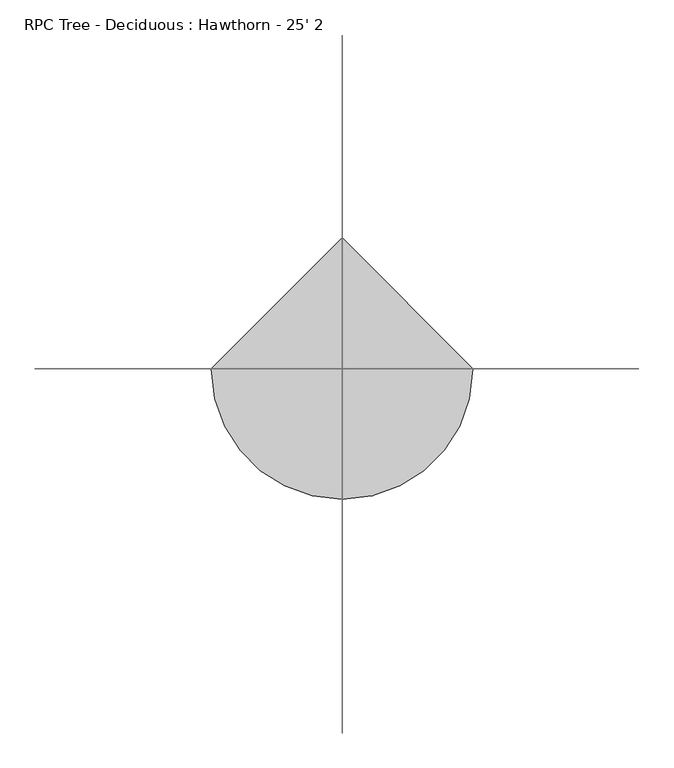
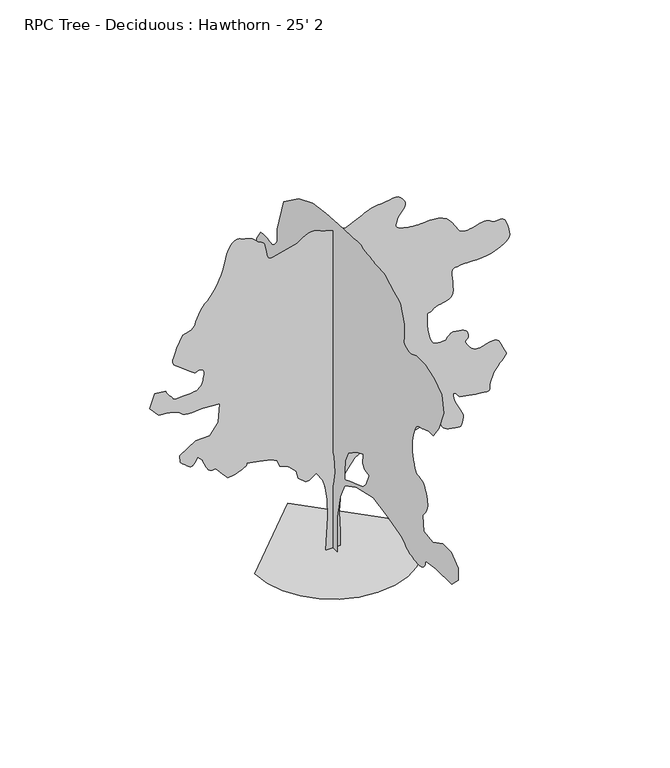
"""IFC4 building model written with IfcOpenShell, lengths in millimetres: geographic element geometry, RPC Tree - Deciduous : Hawthorn - 25' 2."""

from ifc_helpers import new_model, si_unit, origin, place, context, project, spatial, triangles, source, transform, mapped, element, save


def rpc_tree_deciduous_hawthorn_25_2_a438f522(model_context):
    return source(origin(), model_context, "Body", "Tessellation", [
        triangles([(159.1331283, 0.0003947, 0.019308), (-154.090976, 0.0003947, 0.019308), (-109.3440979, 0.0003507, 738.3315319), (-120.5310059, 0.000328, 1118.6758307), (-165.2768666, 0.0003107, 1409.5258827), (-210.0237538, 0.0003, 1588.5119053), (-355.4472356, 0.000288, 1789.8701088), (-500.8748051, 0.000294, 1689.1897717), (-579.1803815, 0.0002947, 1678.0035358), (-735.7915707, 0.0002867, 1812.2424351), (-780.538694, 0.000276, 1991.2284576), (-937.1498468, 0.0002667, 2147.8396832), (-1127.3219599, 0.000262, 2226.1452232), (-1183.2552464, 0.000254, 2360.3841225), (-1306.3080551, 0.00025, 2427.5035721), (-1563.5970016, 0.0002467, 2483.4367859), (-1820.8885643, 0.000244, 2528.1814384), (-1818.86674, 0.0002446, 2518.4962738), (-1819.0953598, 0.0002452, 2508.2221916), (-1823.8248676, 0.0002459, 2496.7743439), (-1835.3057076, 0.0002466, 2483.5664291), (-1855.7857075, 0.0002476, 2468.0089485), (-1887.5203983, 0.0002487, 2449.5176353), (-1932.7551373, 0.00025, 2427.5035721), (-1983.2071449, 0.0002513, 2406.1420853), (-2029.5519905, 0.0002523, 2389.4746433), (-2072.4703011, 0.000253, 2376.7238228), (-2112.6530228, 0.0002536, 2367.102317), (-2150.7784573, 0.000254, 2359.8303772), (-2187.5321732, 0.0002544, 2354.1230221), (-2223.605262, 0.0002547, 2349.1978867), (-2346.6579254, 0.0002467, 2483.4367859), (-2480.8968246, 0.0002373, 2640.0478661), (-2507.2492859, 0.0002376, 2635.5522102), (-2533.5026253, 0.0002377, 2632.8090637), (-2559.5553955, 0.0002377, 2633.596225), (-2585.33638, 0.0002373, 2639.6670753), (-2610.710994, 0.0002366, 2652.7732521), (-2635.5774994, 0.0002353, 2674.6934258), (-2659.885318, 0.0002333, 2707.1548164), (-2681.9072296, 0.0002311, 2744.2133102), (-2700.3982521, 0.000229, 2778.9097389), (-2715.9429428, 0.0002271, 2811.6501823), (-2729.1511482, 0.0002252, 2842.8413017), (-2740.6065536, 0.0002234, 2872.8385986), (-2750.8681366, 0.0002217, 2902.0740234), (-2760.570742, 0.00022, 2930.9030777), (-2861.2308769, 0.000214, 3031.5885017), (-2928.3631165, 0.00022, 2930.9030777), (-2940.4789467, 0.0002211, 2912.005394), (-2953.5089653, 0.0002221, 2894.8857994), (-2968.2664948, 0.0002229, 2881.2968033), (-2985.6907219, 0.0002234, 2872.9656258), (-3006.6202583, 0.0002235, 2871.6956451), (-3031.9695831, 0.0002231, 2879.2396614), (-3062.6020157, 0.000222, 2897.3496025), (-3096.5362816, 0.0002205, 2923.0035599), (-3130.1150459, 0.0002188, 2950.6387917), (-3161.5093506, 0.0002172, 2978.0708382), (-3189.0175552, 0.0002157, 3003.1405289), (-3210.8362816, 0.0002144, 3023.7145638), (-3225.212439, 0.0002136, 3037.6337723), (-3230.3940994, 0.0002133, 3042.7645638), (-3241.5701614, 0.000204, 3199.3808762), (-2905.9857033, 0.0001913, 3411.9277863), (-2603.9547203, 0.0001906, 3423.1038483), (-2424.9634655, 0.0001766, 3658.0281715), (-2391.402578, 0.0001526, 4060.7448692), (-2760.570742, 0.0001506, 4094.2980537), (-2839.3868614, 0.0001512, 4085.027108), (-2916.5522095, 0.0001516, 4077.7374367), (-2990.3898537, 0.0001518, 4074.3338654), (-3059.2490227, 0.0001517, 4076.8229576), (-3121.4283669, 0.0001511, 4087.1354095), (-3175.301532, 0.0001499, 4107.2266251), (-3219.2180374, 0.000148, 4139.0528801), (-3263.4394661, 0.0001459, 4173.1650421), (-3318.227401, 0.0001444, 4199.6317406), (-3381.8287514, 0.0001432, 4219.7741158), (-3452.4660095, 0.0001423, 4234.8106979), (-3528.3866661, 0.0001416, 4246.0120491), (-3607.8379211, 0.0001411, 4254.6990189), (-3689.0413948, 0.0001406, 4262.0904282), (-3879.2111824, 0.000128, 4474.6373383), (-3767.3496964, 0.0001106, 4765.4925499), (-3543.6267242, 0.000112, 4743.1151367), (-3529.174118, 0.0001135, 4716.8007545), (-3514.3404305, 0.0001151, 4690.7657158), (-3498.7195816, 0.0001166, 4665.3402328), (-3481.9046196, 0.0001181, 4640.7786507), (-3463.5406242, 0.0001195, 4617.3853111), (-3443.2206436, 0.0001208, 4595.4904266), (-3420.563887, 0.000122, 4575.3227623), (-3403.5713196, 0.0001231, 4556.2983421), (-3395.5956436, 0.0001242, 4538.2642685), (-3389.1692917, 0.0001251, 4522.1861801), (-3376.875856, 0.0001259, 4509.0544235), (-3351.2727676, 0.0001265, 4499.8340561), (-3304.9177483, 0.0001267, 4495.4907166), (-3230.3940994, 0.0001266, 4497.0147514), (-3147.7933273, 0.0001263, 4501.8153305), (-3080.4326134, 0.0001261, 4506.6159096), (-3025.7972855, 0.0001258, 4511.3911995), (-2981.3473824, 0.0001255, 4516.1917786), (-2944.5429428, 0.0001252, 4520.9923576), (-2912.7928459, 0.0001249, 4525.7929367), (-2883.6082901, 0.0001246, 4530.5679359), (-2855.0332901, 0.0001233, 4552.2596352), (-2827.6521126, 0.000122, 4574.6370483), (-2802.607711, 0.0001206, 4598.3858894), (-2781.0686188, 0.0001191, 4624.1668739), (-2764.2539474, 0.0001174, 4652.7165848), (-2753.2810707, 0.0001154, 4684.6695763), (-2749.3693909, 0.0001133, 4720.7377235), (-2745.4071327, 0.0001109, 4760.7934181), (-2736.720163, 0.0001084, 4802.805098), (-2728.2366692, 0.0001059, 4844.6133018), (-2724.858387, 0.0001036, 4884.0850204), (-2731.4370552, 0.0001015, 4919.0352127), (-2752.8999893, 9.98e-05, 4947.3561584), (-2794.1242172, 9.86e-05, 4966.8636887), (-2835.4754723, 9.84e-05, 4971.2320267), (-2860.596032, 9.89e-05, 4962.0883987), (-2879.2396614, 9.97e-05, 4949.2356949), (-2901.2359932, 0.0001001, 4942.4541321), (-2936.3132126, 9.95e-05, 4951.5216019), (-2994.3015335, 9.75e-05, 4986.2183212), (-3084.9794289, 9.33e-05, 5056.3477615), (-3185.5886948, 8.86e-05, 5134.4522964), (-3266.6398521, 8.52e-05, 5192.2121429), (-3327.7268211, 8.25e-05, 5238.0337646), (-3368.4429405, 7.99e-05, 5280.3497864), (-3388.4327087, 7.71e-05, 5327.5178375), (-3387.2897552, 7.35e-05, 5388.0205399), (-3364.6329987, 6.86e-05, 5470.2399399), (-3332.3750839, 6.34e-05, 5558.3020065), (-3302.4792343, 5.9e-05, 5632.2666779), (-3274.5137901, 5.53e-05, 5694.4966003), (-3248.1488297, 5.21e-05, 5747.3282593), (-3222.926532, 4.94e-05, 5793.1248825), (-3198.4916862, 4.69e-05, 5834.2217926), (-3174.4635017, 4.46e-05, 5872.9566376), (-3129.0991196, 4.4e-05, 5882.81185), (-3084.8015327, 4.34e-05, 5894.2163864), (-3042.6628258, 4.25e-05, 5908.7707306), (-3003.7500847, 4.13e-05, 5928.0236252), (-2969.155394, 3.98e-05, 5953.5255569), (-2939.945549, 3.78e-05, 5986.850267), (-2917.1617653, 3.53e-05, 6029.5732407), (-2900.9310699, 3.27e-05, 6072.7020035), (-2888.6120544, 3.06e-05, 6108.7701508), (-2877.258387, 2.86e-05, 6141.7140701), (-2863.9487343, 2.66e-05, 6175.4195709), (-2845.7370552, 2.43e-05, 6213.8497833), (-2819.7273056, 2.15e-05, 6260.8649368), (-2782.9228661, 1.79e-05, 6320.4281616), (-2744.5688118, 1.47e-05, 6374.7841461), (-2713.0727692, 1.26e-05, 6410.1918686), (-2684.3201637, 1.1e-05, 6436.3792236), (-2654.1702599, 9.4e-06, 6463.150264), (-2618.5596428, 7.2e-06, 6500.2852066), (-2573.3475769, 3.8e-06, 6557.5875229), (-2514.4552414, -1.4e-06, 6644.8362671), (-2453.8586494, -7.4e-06, 6746.4620407), (-2405.0042187, -1.31e-05, 6841.4324066), (-2365.9314583, -1.85e-05, 6931.32285), (-2334.6868538, -2.36e-05, 7017.682695), (-2309.3123852, -2.86e-05, 7102.0868454), (-2287.8543926, -3.36e-05, 7186.1102051), (-2268.3497692, -3.87e-05, 7271.2759369), (-2244.5754936, -4.38e-05, 7356.7980423), (-2212.386034, -4.86e-05, 7437.6204346), (-2172.9551559, -5.29e-05, 7509.0451447), (-2127.4586597, -5.63e-05, 7566.3730408), (-2077.0701656, -5.86e-05, 7604.9299896), (-2022.9657646, -5.95e-05, 7619.9924423), (-1966.3136993, -5.87e-05, 7606.8862656), (-1910.121199, -5.73e-05, 7582.9086594), (-1856.4689507, -5.63e-05, 7565.7887741), (-1805.1685936, -5.54e-05, 7551.412326), (-1756.0195587, -5.45e-05, 7535.6644501), (-1708.8265091, -5.32e-05, 7514.4302811), (-1663.3961426, -5.14e-05, 7483.5943726), (-1619.5303608, -4.87e-05, 7439.0936005), (-1579.0555058, -4.63e-05, 7399.0890656), (-1543.670747, -4.51e-05, 7378.0827896), (-1512.9800331, -4.44e-05, 7366.2974625), (-1486.5970505, -4.37e-05, 7353.9022888), (-1464.1256023, -4.23e-05, 7331.1437943), (-1445.1773403, -3.97e-05, 7288.217926), (-1429.3581024, -3.54e-05, 7215.3456299), (-1415.9875523, -3.04e-05, 7132.3890656), (-1403.2038849, -2.64e-05, 7065.2571167), (-1388.8528713, -2.34e-05, 7013.4155136), (-1370.7858055, -2.11e-05, 6976.2299927), (-1346.8464237, -1.98e-05, 6953.1412857), (-1314.8855839, -1.92e-05, 6943.5401276), (-1272.7470222, -1.94e-05, 6946.8678314), (-758.1663677, -2.74e-05, 7081.1067307), (-698.2198814, -2.99e-05, 7123.7785446), (-638.1794329, -3.23e-05, 7163.5040268), (-577.9408496, -3.43e-05, 7197.3368454), (-517.4101693, -3.58e-05, 7222.4068268), (-456.4857994, -3.66e-05, 7235.6908997), (-395.0737412, -3.65e-05, 7234.3444702), (-333.0749456, -3.54e-05, 7215.3456299), (-271.7289263, -3.38e-05, 7188.8786407), (-212.1431193, -3.25e-05, 7166.5015182), (-154.0251915, -3.14e-05, 7147.5526749), (-97.0814925, -3.04e-05, 7131.34785), (-41.0181631, -2.95e-05, 7117.1742966), (14.4578691, -2.88e-05, 7104.3983322), (69.6403804, -2.81e-05, 7092.3077911), (270.9999556, -2.67e-05, 7069.9306686), (584.2222612, -3.47e-05, 7204.1695679), (629.9473045, -3.64e-05, 7232.7445679), (676.749317, -3.81e-05, 7260.1254547), (725.7026516, -3.96e-05, 7285.1698563), (777.8843502, -4.08e-05, 7306.7092392), (834.371382, -4.18e-05, 7323.5239105), (896.2406433, -4.25e-05, 7334.4964966), (964.56656, -4.27e-05, 7338.4084671), (1038.7294024, -4.3e-05, 7343.6912842), (1115.4373655, -4.38e-05, 7356.0102997), (1191.7540735, -4.46e-05, 7370.107695), (1264.743441, -4.52e-05, 7380.6739105), (1331.4717808, -4.54e-05, 7382.4261292), (1389.0027168, -4.46e-05, 7370.107695), (1434.402562, -4.27e-05, 7338.4084671), (1469.8203129, -4.03e-05, 7297.1080811), (1498.5858536, -3.8e-05, 7258.7540268), (1519.5229477, -3.58e-05, 7222.177771), (1531.4610271, -3.37e-05, 7186.1607834), (1533.2212395, -3.15e-05, 7149.5595291), (1523.6327259, -2.92e-05, 7111.2054749), (1501.5195408, -2.67e-05, 7069.9306686), (1474.1255733, -2.45e-05, 7032.3637756), (1449.4698109, -2.28e-05, 7003.585881), (1427.5522533, -2.14e-05, 6980.1163834), (1408.3752262, -2.01e-05, 6958.3991043), (1391.9388748, -1.87e-05, 6934.9040268), (1378.2407284, -1.7e-05, 6906.151712), (1367.2806416, -1.47e-05, 6868.5598206), (1355.7362881, -1.23e-05, 6828.0210159), (1343.4097149, -1.02e-05, 6792.1819244), (1334.9946762, -8.3e-06, 6760.2542221), (1335.1903038, -6.6e-06, 6731.4507477), (1348.692968, -5e-06, 6705.0093384), (1380.1965683, -3.5e-06, 6680.1172531), (1434.402562, -2.1e-06, 6656.0123291), (1502.5633724, -8e-07, 6635.3118484), (1571.509164, 1e-07, 6620.4778702), (1639.2813354, 7e-07, 6610.5209198), (1703.9217213, 1e-06, 6604.5015198), (1763.4744816, 1.2e-06, 6601.4028717), (1815.9839218, 1.3e-06, 6600.2593369), (1859.4914406, 1.3e-06, 6600.0820221), (1908.6404755, 1.1e-06, 6602.7998795), (1975.9885448, 8e-07, 6608.0571167), (2056.4454071, 6e-07, 6611.5371368), (2144.9261982, 8e-07, 6608.9715958), (2236.3432926, 1.5e-06, 6596.0177353), (2325.6064487, 3.2e-06, 6568.3827942), (2407.633128, 5.9e-06, 6521.7734299), (2476.0555504, 9.6e-06, 6460.1789337), (2530.3911873, 1.36e-05, 6393.2754593), (2574.3635033, 1.77e-05, 6325.4063461), (2611.6760513, 2.15e-05, 6260.8649368), (2646.0422676, 2.49e-05, 6203.9689911), (2681.1959358, 2.76e-05, 6158.9856903), (2720.8452599, 2.93e-05, 6130.258374), (2765.3207428, 3.01e-05, 6115.9580841), (2812.1074219, 3.05e-05, 6110.4973709), (2860.8753754, 3.04e-05, 6112.3513275), (2911.1926529, 2.99e-05, 6120.0729492), (2962.6784637, 2.92e-05, 6132.2140686), (3014.9770157, 2.83e-05, 6147.2765213), (3067.6310692, 2.73e-05, 6163.8115585), (3115.4592545, 2.67e-05, 6173.1080841), (3162.4746986, 2.63e-05, 6180.6518097), (3207.9405281, 2.6e-05, 6184.6649368), (3251.0698723, 2.61e-05, 6183.3952469), (3291.0494087, 2.66e-05, 6175.0637787), (3327.1172653, 2.76e-05, 6157.9444748), (3358.4862808, 2.93e-05, 6130.258374), (3393.4620529, 3.05e-05, 6109.9386841), (3438.1912994, 3.06e-05, 6108.7957306), (3488.8135002, 3.01e-05, 6115.881926), (3541.3913956, 2.99e-05, 6120.200267), (3592.0135963, 3.04e-05, 6110.8531631), (3636.7428429, 3.25e-05, 6076.8424484), (3671.718615, 3.66e-05, 6007.1955368), (3699.2776886, 4.18e-05, 5920.2258453), (3722.3408157, 4.65e-05, 5841.4608856), (3737.75877, 5.07e-05, 5770.9250748), (3742.4323219, 5.44e-05, 5708.5934143), (3733.1866653, 5.76e-05, 5654.4914841), (3706.9484413, 6.04e-05, 5608.5937042), (3660.5172638, 6.26e-05, 5570.9256546), (3605.0439056, 6.46e-05, 5537.5247864), (3550.9419754, 6.65e-05, 5505.1145554), (3494.096608, 6.84e-05, 5474.6594376), (3430.3935196, 7e-05, 5447.1262344), (3355.7431343, 7.14e-05, 5423.5044205), (3266.0302963, 7.25e-05, 5404.7846329), (3157.1407219, 7.33e-05, 5391.931929), (3050.6893707, 7.37e-05, 5385.4549988), (2967.1235413, 7.38e-05, 5383.8550964), (2900.6008575, 7.37e-05, 5385.2009445), (2845.2036575, 7.36e-05, 5387.5124313), (2795.1148544, 7.35e-05, 5388.8332809), (2744.4417847, 7.36e-05, 5387.2327972), (2687.2917847, 7.4e-05, 5380.755867), (2632.1995079, 7.44e-05, 5373.8725662), (2590.4418823, 7.46e-05, 5369.5292267), (2560.1905312, 7.5e-05, 5363.4330872), (2539.7510811, 7.57e-05, 5351.2663879), (2527.325386, 7.71e-05, 5328.7369492), (2521.1609367, 7.93e-05, 5291.5258484), (2519.4970848, 8.26e-05, 5235.3409058), (2523.9979729, 8.71e-05, 5159.8269104), (2533.5866318, 9.23e-05, 5072.4002701), (2542.3849319, 9.78e-05, 4980.2494995), (2544.5441025, 0.0001032, 4890.6636887), (2534.1732239, 0.0001079, 4810.8569321), (2505.4078285, 0.0001117, 4748.0680321), (2452.3776352, 0.000114, 4709.5616615), (2387.9658691, 0.0001152, 4689.2416809), (2328.8373562, 0.0001161, 4674.4079933), (2274.7963234, 0.0001168, 4662.2924538), (2225.6474339, 0.0001175, 4650.2019127), (2181.1949146, 0.0001184, 4635.3682251), (2141.2406673, 0.0001196, 4615.0482445), (2105.594442, 0.0001213, 4586.4988243), (2074.7410927, 0.0001226, 4564.2231491), (2049.1734673, 0.000123, 4557.6189011), (2028.6908512, 0.0001231, 4556.2727623), (2013.1029945, 0.0001235, 4549.846701), (2002.2088921, 0.0001248, 4527.9773964), (1995.8156776, 0.0001276, 4480.2506584), (1993.727869, 0.0001326, 4396.3293274), (1998.2947414, 0.000139, 4289.0143661), (2011.0810249, 0.0001454, 4181.4709305), (2030.7126755, 0.0001515, 4079.0327065), (2055.8256775, 0.000157, 3986.9578033), (2085.0483124, 0.0001616, 3910.5546181), (2117.0091522, 0.0001649, 3855.0812599), (2150.3415653, 0.0001666, 3825.8202553), (2188.6294899, 0.0001673, 3814.6444839), (2233.3766132, 0.0001676, 3808.9294258), (2280.0795765, 0.0001677, 3807.3292328), (2324.2399624, 0.0001677, 3808.4721863), (2361.351796, 0.0001675, 3810.9868584), (2386.9220375, 0.0001674, 3813.5015305), (2396.4468922, 0.0001673, 3814.6444839), (2400.0004543, 0.0001668, 3823.2041359), (2411.1865448, 0.0001655, 3844.8958351), (2430.787674, 0.0001638, 3873.6231514), (2459.5862068, 0.000162, 3903.3411049), (2498.3643631, 0.0001605, 3927.9791359), (2547.8968048, 0.0001597, 3941.4411049), (2608.9837738, 0.00016, 3937.6817413), (2671.9758591, 0.0001607, 3924.8296188), (2726.5347382, 0.0001614, 3912.9675522), (2772.483387, 0.0001623, 3898.9468964), (2809.6183296, 0.0001634, 3879.6428421), (2837.7866684, 0.0001651, 3851.906163), (2856.7352211, 0.0001674, 3812.6379204), (2866.2855103, 0.0001706, 3758.7135956), (2862.7040428, 0.0001735, 3709.9456421), (2847.1593521, 0.0001752, 3682.3104103), (2826.9411095, 0.0001761, 3666.8418777), (2809.2625374, 0.0001769, 3654.4722839), (2801.3885994, 0.0001779, 3636.235025), (2810.5072289, 0.0001799, 3603.1387894), (2843.9080971, 0.0001833, 3546.1666855), (2889.3486374, 0.000187, 3484.6480568), (2930.6490234, 0.0001895, 3441.7218979), (2969.2315521, 0.0001912, 3414.061377), (3006.467942, 0.0001921, 3398.3640793), (3043.6790428, 0.0001925, 3391.2523041), (3082.2615715, 0.0001926, 3389.4233459), (3123.5619576, 0.0001926, 3389.5503731), (3174.7428452, 0.0001921, 3399.3294273), (3238.4459335, 0.0001908, 3421.249601), (3309.3628258, 0.0001894, 3444.134832), (3382.2607018, 0.0001886, 3456.860218), (3451.8311646, 0.0001891, 3448.2496971), (3512.7911064, 0.0001916, 3407.1524963), (3559.8571289, 0.0001966, 3322.4181335), (3596.9920715, 0.0002022, 3228.6924591), (3629.6310677, 0.0002061, 3162.9572273), (3654.6498894, 0.0002089, 3117.5419762), (3668.8993103, 0.0002108, 3084.8776909), (3669.2803917, 0.0002124, 3057.2680389), (3652.5924568, 0.0002142, 3027.1437149), (3615.7880173, 0.0002166, 2986.8336754), (3572.5063568, 0.0002193, 2942.3837723), (3537.6831917, 0.0002217, 2904.233194), (3509.8447746, 0.0002237, 2871.3148544), (3487.6196777, 0.0002256, 2842.5872475), (3469.6111839, 0.0002272, 2817.0094482), (3454.4219948, 0.0002288, 2793.5399506), (3440.6298134, 0.0002303, 2771.0863792), (3437.2006622, 0.00023, 2773.5501823), (3432.5271103, 0.0002299, 2772.1278854), (3425.3897552, 0.0002303, 2763.0345451), (3414.5439056, 0.0002314, 2742.4099319), (3398.7451607, 0.0002335, 2706.4182335), (3376.7235397, 0.0002367, 2651.1986389), (3347.3102188, 0.0002413, 2572.9412064), (3325.1359909, 0.0002461, 2493.0582916), (3319.1924583, 0.0002496, 2433.9271626), (3319.7005669, 0.000252, 2392.9976841), (3316.9065514, 0.0002535, 2367.722192), (3300.9807793, 0.0002543, 2355.5581089), (3262.1694855, 0.0002544, 2353.9579159), (3190.6939064, 0.000254, 2360.3841225), (3103.5213203, 0.0002534, 2370.2977615), (3023.3843513, 0.0002528, 2380.8006088), (2949.1147568, 0.0002521, 2391.791217), (2879.544294, 0.0002514, 2403.1729351), (2813.5044296, 0.0002507, 2414.8492573), (2749.8266304, 0.00025, 2426.721207), (2687.2917847, 0.0002493, 2438.6895172), (2647.0584846, 0.0002464, 2487.937674), (2609.8473839, 0.0002438, 2530.6275101), (2578.6815536, 0.0002421, 2560.2158203), (2556.6343529, 0.0002415, 2570.1219017), (2546.7285622, 0.0002425, 2553.8150482), (2551.9863808, 0.0002454, 2504.7319977), (2575.4302986, 0.0002507, 2416.3173363), (2612.9463226, 0.0002568, 2313.8436493), (2654.9324226, 0.000262, 2225.2638817), (2696.3598358, 0.0002666, 2148.0351654), (2732.09748, 0.0002707, 2079.6102722), (2757.0910126, 0.0002744, 2017.4488049), (2766.209642, 0.0002779, 1959.0060059), (2754.4240242, 0.0002813, 1901.734211), (2736.8980591, 0.0002844, 1850.8910934), (2728.0081947, 0.0002866, 1812.7631882), (2721.2516304, 0.0002882, 1786.3802055), (2710.2025955, 0.0002891, 1770.7567406), (2688.3841599, 0.0002895, 1764.9197422), (2649.3443916, 0.0002893, 1767.8864216), (2586.6063606, 0.0002887, 1778.6815475), (2516.4972679, 0.0002878, 1792.6413059), (2458.5092377, 0.000287, 1806.7966919), (2411.0875683, 0.000286, 1822.7122902), (2372.6700005, 0.0002849, 1841.9528309), (2341.6871532, 0.0002834, 1866.0878403), (2316.5741512, 0.0002816, 1896.6795776), (2295.766555, 0.0002793, 1935.2952438), (2282.6220085, 0.0002768, 1976.9435738), (2278.2862267, 0.0002746, 2015.0688629), (2277.8621246, 0.0002726, 2048.8888916), (2276.46003, 0.0002708, 2077.6214401), (2269.185474, 0.0002695, 2100.4838528), (2251.1515457, 0.0002685, 2116.6915844), (2217.4610149, 0.000268, 2125.4673569), (2177.5728973, 0.0002678, 2129.2823856), (2143.5572411, 0.0002676, 2131.3372021), (2114.4335827, 0.0002676, 2131.9239395), (2089.2216042, 0.0002676, 2131.3372021), (2066.9483997, 0.0002677, 2129.8691231), (2046.6284191, 0.0002678, 2127.8143066), (2027.2887566, 0.000268, 2125.4673569), (1758.8111034, 0.000274, 2024.7868744), (1579.8250809, 0.0002667, 2147.8396832), (1380.9128036, 0.0002704, 2075.457328), (1410.85429, 0.0002716, 2057.3014595), (1436.60984, 0.0002729, 2038.5130714), (1453.9936626, 0.0002741, 2018.4597897), (1458.8195309, 0.0002755, 1996.5066238), (1446.9019444, 0.0002771, 1972.0210545), (1414.0572922, 0.0002788, 1944.370562), (1356.0970219, 0.0002807, 1912.9203014), (1293.4784603, 0.0002823, 1885.3308517), (1245.5334217, 0.0002833, 1868.8920296), (1206.3972204, 0.0002837, 1862.4353016), (1170.1971771, 0.0002835, 1864.7822514), (1131.0609032, 0.0002829, 1874.7644909), (1083.118408, 0.0002819, 1891.2008423), (1020.4998465, 0.0002807, 1912.9203014), (729.6473236, 0.0002753, 2002.4145481), (461.1695615, 0.000284, 1856.9895584), (259.8112671, 0.0003, 1588.5119053), (192.6930892, 0.0003113, 1398.3397923), (170.3192732, 0.0003253, 1163.422954), (136.7603205, 0.0003487, 771.8924921), (159.1331283, 0.0003767, 302.0564901), (-0.000123, -157.488225, 0.0160584), (-0.000123, 166.924822, 0.0160778), (-0.0001013, 177.738606, 702.9113102), (-8.68e-05, 231.8072715, 1059.765691), (-7.23e-05, 404.8273247, 1416.6200718), (-6.51e-05, 567.0341025, 1654.5213936), (-5.79e-05, 848.1915413, 1849.1689602), (-4.34e-05, 1334.8118385, 2065.4447124), (-2.89e-05, 1907.9419716, 2130.3263626), (-2.89e-05, 2243.1683121, 1924.8659386), (-2.89e-05, 2491.8848167, 1892.4250408), (-2.17e-05, 2632.4532715, 2162.7697311), (-1.45e-05, 2859.5545258, 2195.2106289), (-7.2e-06, 3335.3469955, 2227.6513813), (0.0, 3616.5246002, 2249.279567), (7.2e-06, 3757.0881134, 2357.4172977), (7.2e-06, 3746.2931328, 2530.436824), (1.45e-05, 3919.2921661, 2638.5747002), (1.45e-05, 3967.7046181, 2647.972673), (1.45e-05, 4014.4912971, 2658.1328087), (1.45e-05, 4058.052301, 2669.7913994), (2.17e-05, 4096.7874367, 2683.7106079), (2.17e-05, 4129.1215096, 2700.6775955), (2.17e-05, 4153.3784592, 2721.4295265), (2.17e-05, 4168.0089615, 2746.7024025), (2.17e-05, 4176.6447716, 2777.0299118), (2.17e-05, 4184.163208, 2811.9042366), (2.17e-05, 4190.7162964, 2850.5629234), (2.89e-05, 4196.5075127, 2892.2443909), (2.89e-05, 4201.7400421, 2936.1861855), (2.89e-05, 4206.6167793, 2981.6523056), (2.89e-05, 4211.2650421, 3027.8802979), (3.62e-05, 4027.4454483, 3254.9559723), (2.89e-05, 3627.3195808, 3276.5968025), (2.17e-05, 3389.4233459, 3103.5721893), (2.17e-05, 3374.8945816, 3100.7020157), (2.17e-05, 3336.7184235, 3093.8440041), (2.17e-05, 3283.0228638, 3085.690432), (1.45e-05, 3221.9614746, 3078.8580002), (1.45e-05, 3161.6363777, 3075.9878265), (1.45e-05, 3110.2270157, 3079.7216103), (1.45e-05, 3075.8352196, 3092.7516289), (1.45e-05, 3052.3404327, 3114.7479607), (1.45e-05, 3028.2866684, 3143.0183281), (1.45e-05, 3003.7500847, 3176.4444855), (1.45e-05, 2978.8582901, 3214.0619568), (2.17e-05, 2953.6615723, 3254.803656), (2.17e-05, 2928.2869583, 3297.6277863), (2.17e-05, 2902.8106064, 3341.4681335), (2.89e-05, 2848.734256, 3611.8254684), (3.62e-05, 3075.8352196, 3784.8247925), (5.06e-05, 3248.8598328, 4076.7976685), (5.06e-05, 2967.6822281, 4336.3344429), (4.34e-05, 2675.7096428, 4239.0017212), (3.62e-05, 2491.8848167, 4087.6179382), (3.62e-05, 2286.4219219, 4228.2067406), (4.34e-05, 2286.4219219, 4466.1029755), (5.79e-05, 2481.0694885, 4682.3836693), (5.79e-05, 2522.6544502, 4705.5229546), (5.79e-05, 2563.4923645, 4728.4593452), (5.79e-05, 2602.786187, 4751.0399437), (5.79e-05, 2639.8446808, 4773.0362755), (5.79e-05, 2673.8553955, 4794.2960243), (6.51e-05, 2704.0811668, 4814.5907158), (6.51e-05, 2729.7859932, 4833.7674522), (6.51e-05, 2749.8013412, 4860.5137848), (6.51e-05, 2764.1522095, 4901.992067), (6.51e-05, 2773.7789474, 4955.7887833), (7.23e-05, 2779.5954529, 5019.390715), (7.23e-05, 2782.5926537, 5090.4090546), (7.23e-05, 2783.710318, 5166.3038406), (7.23e-05, 2783.8626343, 5244.688591), (7.96e-05, 2643.2738319, 5460.9689941), (7.96e-05, 2638.1936188, 5462.1375275), (7.96e-05, 2623.8680397, 5465.0077011), (7.96e-05, 2601.5670753, 5468.6400375), (7.96e-05, 2572.6618629, 5472.068898), (7.96e-05, 2538.4505791, 5474.354805), (7.96e-05, 2500.2694794, 5474.5832794), (7.96e-05, 2459.4440643, 5471.7892639), (7.96e-05, 2416.0634274, 5465.5158096), (7.23e-05, 2370.5999233, 5457.3366577), (7.23e-05, 2324.9486401, 5449.3615631), (7.23e-05, 2281.0014679, 5443.6462143), (7.23e-05, 2240.6460823, 5442.3003662), (7.23e-05, 2205.7769897, 5447.3802887), (7.23e-05, 2178.2865166, 5460.9689941), (7.23e-05, 2156.0590942, 5480.4509445), (7.23e-05, 2135.5359283, 5501.6345352), (7.23e-05, 2116.4299725, 5524.2407135), (7.23e-05, 2098.4595577, 5547.9892639), (7.23e-05, 2081.3399632, 5572.5767166), (7.23e-05, 2064.7867584, 5597.7228561), (7.23e-05, 2048.5206001, 5623.1736282), (8.68e-05, 2037.7052719, 5893.5053833), (0.0001013, 1810.6168076, 6650.4754578), (0.0001085, 1259.1148602, 7050.6010345), (0.0001085, 740.0536652, 7266.8564392), (0.0001013, 264.2486416, 7331.7536407), (9.4e-05, -200.7431066, 7364.1894516), (8.68e-05, -654.9205622, 7385.8299911), (8.68e-05, -694.7400793, 7388.0908997), (8.68e-05, -753.6629362, 7393.3737167), (8.68e-05, -824.3155277, 7399.4442764), (8.68e-05, -899.3190891, 7403.9655121), (8.68e-05, -971.295001, 7404.7276749), (7.96e-05, -1032.8671148, 7399.4442764), (7.96e-05, -1076.6592093, 7385.8299911), (7.96e-05, -1121.7111105, 7368.5327911), (7.96e-05, -1186.8138227, 7353.5464966), (7.96e-05, -1264.2126595, 7340.41474), (7.96e-05, -1346.1503906, 7328.807309), (7.23e-05, -1424.8724751, 7318.3422501), (7.23e-05, -1492.6244442, 7308.6393539), (7.23e-05, -1541.6489227, 7299.3178299), (7.23e-05, -1586.6069344, 7292.8658981), (7.23e-05, -1644.4273876, 7290.2247803), (7.23e-05, -1710.7593853, 7288.5225586), (6.51e-05, -1781.254501, 7284.9413818), (6.51e-05, -1851.5590759, 7276.6099136), (6.51e-05, -1917.3246838, 7260.7097214), (6.51e-05, -1974.2002819, 7234.4206284), (6.51e-05, -2029.2775887, 7201.04534), (5.79e-05, -2091.7336601, 7165.9422501), (5.79e-05, -2160.3364494, 7129.4427338), (5.79e-05, -2233.8566711, 7091.7996826), (5.06e-05, -2311.0675106, 7053.2933121), (5.06e-05, -2390.7344501, 7014.2282547), (5.06e-05, -2471.6334366, 6974.8835632), (3.62e-05, -2623.0300095, 6596.4241058), (2.17e-05, -2612.209449, 6250.3748795), (2.17e-05, -2603.3448738, 6234.0683167), (2.17e-05, -2596.9441017, 6217.3042236), (2.17e-05, -2595.4709358, 6199.5750732), (2.17e-05, -2601.3638901, 6180.4489151), (2.17e-05, -2617.1117661, 6159.4176407), (2.17e-05, -2645.1280792, 6136.0243011), (2.17e-05, -2687.9016312, 6109.7863678), (2.17e-05, -2739.2095459, 6088.9329895), (1.45e-05, -2791.0761475, 6080.5253632), (1.45e-05, -2843.4002792, 6082.5572159), (1.45e-05, -2896.1052017, 6092.894957), (1.45e-05, -2949.1147568, 6109.4811539), (1.45e-05, -3002.3024986, 6130.2327942), (1.45e-05, -3055.5661079, 6153.0424484), (7.2e-06, -3390.7950645, 6153.0424484), (0.0, -3726.0237305, 6044.9147461), (-7.2e-06, -3996.3810654, 5850.2743011), (-2.17e-05, -4061.2526871, 5471.7892639), (-2.89e-05, -3877.4330933, 5017.6123352), (-3.62e-05, -3682.7676498, 4747.255291), (-3.62e-05, -3647.7410088, 4747.0773949), (-3.62e-05, -3611.1144653, 4745.7565453), (-3.62e-05, -3571.261956, 4742.1497887), (-3.62e-05, -3526.5832878, 4735.1647499), (-3.62e-05, -3475.4785583, 4723.6078972), (-3.62e-05, -3416.3472839, 4706.4121445), (-2.89e-05, -3347.5389839, 4682.3836693), (-2.89e-05, -3278.5272079, 4659.244384), (-2.89e-05, -3219.1674591, 4642.9122414), (-2.89e-05, -3168.4943893, 4629.6025887), (-2.89e-05, -3125.5938103, 4615.5310638), (-2.89e-05, -3089.5003738, 4596.9383034), (-2.89e-05, -3059.2746025, 4570.0143654), (-2.89e-05, -3033.9508575, 4530.9745972), (-3.62e-05, -3009.1605103, 4474.9675507), (-3.62e-05, -2982.6935211, 4403.2379173), (-3.62e-05, -2956.7602203, 4321.29757), (-3.62e-05, -2933.6970932, 4234.6330925), (-4.34e-05, -2915.7138885, 4148.7301964), (-4.34e-05, -2905.1220932, 4069.0504669), (-4.34e-05, -2904.182325, 4001.1054863), (-5.06e-05, -2913.1739273, 3931.6111816), (-5.06e-05, -2929.7092552, 3849.0868584), (-5.06e-05, -2952.1375374, 3761.6346382), (-5.79e-05, -2978.7056831, 3677.3828041), (-5.79e-05, -3007.7379227, 3604.510508), (-6.51e-05, -3037.5320343, 3551.0942917), (-6.51e-05, -3066.3866684, 3525.3133072), (-6.51e-05, -3100.752594, 3518.1250832), (-6.51e-05, -3145.3295242, 3512.8163956), (-6.51e-05, -3195.7741196, 3506.0092529), (-6.51e-05, -3247.7424591, 3494.2745041), (-6.51e-05, -3296.840625, 3474.2338669), (-7.23e-05, -3338.775856, 3442.4584808), (-7.23e-05, -3369.1795235, 3395.5447746), (-7.23e-05, -3392.7507591, 3341.163501), (-7.23e-05, -3416.1440987, 3288.8393692), (-7.96e-05, -3437.8357979, 3238.0648521), (-7.96e-05, -3456.3268204, 3188.2048141), (-7.96e-05, -3470.0684235, 3138.7511467), (-7.96e-05, -3477.5612801, 3089.0940033), (-8.68e-05, -3477.3072258, 3038.6752785), (-8.68e-05, -3468.5696777, 2989.2721893), (-8.68e-05, -3452.4660095, 2942.7139847), (-8.68e-05, -3430.2159142, 2898.5181358), (-8.68e-05, -3403.0379219, 2856.2018234), (-8.68e-05, -3372.1767242, 2815.3078079), (-8.68e-05, -3338.8520142, 2775.3791405), (-8.68e-05, -3304.2826126, 2735.9074219), (-0.0001013, -3325.9234428, 2389.8581955), (-0.0001085, -3671.9726692, 2346.6021149), (-0.0001085, -4028.8168762, 2530.436824), (-0.0001085, -4342.4050026, 2530.436824), (-0.000123, -4591.1215073, 2324.9765453), (-0.0001302, -4601.9420677, 2065.4447124), (-0.0001302, -4353.225563, 1827.5433907), (-0.000123, -3769.2801018, 1816.7280624), (-0.000123, -3401.6153343, 1762.6591244), (-0.000123, -3391.887149, 1716.5988544), (-0.000123, -3379.2887901, 1672.2403702), (-0.000123, -3361.0515312, 1631.287928), (-0.000123, -3334.2802002, 1595.4409882), (-0.000123, -3296.1546204, 1566.4036617), (-0.000123, -3243.8560684, 1545.8804958), (-0.000123, -3174.5396599, 1535.57066), (-0.000123, -3100.1939072, 1534.0567989), (-0.000123, -3033.9761467, 1538.0293762), (-0.000123, -2974.7687141, 1546.3529961), (-0.0001157, -2921.4289467, 1557.8922626), (-0.0001157, -2872.8133095, 1571.5116348), (-0.0001157, -2827.8044289, 1586.0760075), (-0.0001157, -2785.2343529, 1600.4524555), (-0.0001157, -2741.7495071, 1620.3151966), (-0.0001157, -2695.6229622, 1649.4464127), (-0.0001085, -2648.1758583, 1683.8735264), (-0.0001085, -2600.7287544, 1719.6265766), (-0.0001085, -2554.6025002, 1752.7277538), (-0.0001085, -2511.138002, 1779.2123291), (-0.0001085, -2471.6334366, 1795.1000221), (-9.4e-05, -1963.3875698, 1935.6812668), (-8.68e-05, -1487.5799847, 2022.1911026), (-7.96e-05, -849.5682014, 1870.7970005), (-7.96e-05, -427.8320978, 1643.7085361), (-8.68e-05, -265.62532, 1308.4821957), (-0.0001013, -157.488225, 789.4210733), (-0.0001157, -157.488225, 356.8696415), (7.2e-06, 350.7584229, 2173.5824432), (7.2e-06, 383.199248, 1989.7475887), (0.0, 350.7584229, 1751.8464123), (-1.45e-05, 220.9934875, 1513.9426197), (-2.17e-05, 69.6010114, 1178.7162792), (-2.17e-05, -27.7230557, 1438.2456413), (-7.2e-06, -81.7917281, 1741.0310841), (0.0, -49.3503716, 2065.4447124), (7.2e-06, 69.6010114, 2314.1612171), (1.45e-05, 177.738606, 2400.6709076), (-3.62e-05, -1109.1000343, 2768.3432327), (-3.62e-05, -860.3835297, 2660.1902412), (-3.62e-05, -568.410799, 2465.5553192), (-4.34e-05, -460.2729229, 2227.6513813), (-5.06e-05, -438.6448462, 1978.9348766), (-5.79e-05, -438.6448462, 1795.1000221), (-5.79e-05, -611.6669523, 1859.9842884), (-5.79e-05, -903.6371395, 1957.3068363), (-5.79e-05, -1109.1000343, 2043.8191429), (-5.79e-05, -1217.2379105, 2162.7697311), (-5.06e-05, -1325.3757866, 2411.4862358), (-4.34e-05, -1163.1689724, 2454.739991), (-4.34e-05, -1098.2847061, 2562.8828087), (-1650.2489799, 0.0, 9.84e-05), (-1606.6219917, -378.1268832, 7.58e-05), (-1482.373035, -725.3775261, 5.51e-05), (-1287.4484505, -1031.8003195, 3.69e-05), (-1031.8003195, -1287.4484505, 2.16e-05), (-725.3775261, -1482.3704189, 1e-05), (-378.1268832, -1606.6219917, 2.6e-06), (6.51e-05, -1650.2489799, 0.0), (378.1268832, -1606.6219917, 2.6e-06), (725.3775261, -1482.3704189, 1e-05), (1031.8003195, -1287.4484505, 2.16e-05), (1287.4484505, -1031.8003195, 3.69e-05), (1482.3704189, -725.3775261, 5.51e-05), (1606.6219917, -378.1268832, 7.58e-05), (1650.2489799, 0.0001443, 9.84e-05), (-0.0002242, 1650.2489799, 0.0001967)], [[403, 404, 405], [1, 2, 3], [491, 1, 3], [490, 491, 3], [490, 3, 4], [489, 490, 4], [489, 4, 5], [488, 489, 5], [84, 85, 86], [84, 86, 87], [83, 84, 87], [83, 87, 88], [83, 88, 89], [83, 89, 90], [82, 83, 90], [82, 90, 91], [82, 91, 92], [81, 82, 92], [81, 92, 93], [81, 93, 94], [81, 94, 95], [81, 95, 96], [81, 96, 97], [80, 81, 97], [80, 97, 98], [79, 80, 98], [79, 98, 99], [78, 79, 99], [78, 99, 100], [77, 78, 100], [77, 100, 101], [488, 5, 6], [487, 488, 6], [76, 77, 101], [76, 101, 102], [75, 76, 102], [74, 75, 102], [73, 74, 102], [73, 102, 103], [72, 73, 103], [72, 103, 104], [71, 72, 104], [71, 104, 105], [70, 71, 105], [70, 105, 106], [70, 106, 107], [69, 70, 107], [68, 69, 107], [68, 107, 108], [68, 108, 109], [68, 109, 110], [68, 110, 111], [68, 111, 112], [63, 64, 65], [62, 63, 65], [61, 62, 65], [60, 61, 65], [59, 60, 65], [58, 59, 65], [57, 58, 65], [56, 57, 65], [55, 56, 65], [54, 55, 65], [53, 54, 65], [52, 53, 65], [51, 52, 65], [50, 51, 65], [49, 50, 65], [48, 49, 65], [48, 65, 66], [47, 48, 66], [30, 31, 32], [467, 468, 469], [487, 6, 7], [486, 487, 7], [68, 112, 113], [8, 9, 10], [7, 8, 10], [7, 10, 11], [29, 30, 32], [414, 415, 416], [414, 416, 417], [413, 414, 417], [413, 417, 418], [412, 413, 418], [412, 418, 419], [141, 142, 143], [411, 412, 419], [411, 419, 420], [12, 13, 14], [28, 29, 32], [424, 425, 426], [27, 28, 32], [442, 443, 444], [441, 442, 444], [441, 444, 445], [440, 441, 445], [440, 445, 446], [439, 440, 446], [439, 446, 447], [438, 439, 447], [437, 438, 447], [436, 437, 447], [436, 447, 448], [435, 436, 448], [435, 448, 449], [435, 449, 450], [435, 450, 451], [435, 451, 452], [435, 452, 453], [435, 453, 454], [435, 454, 455], [435, 455, 456], [434, 435, 456], [434, 456, 457], [433, 434, 457], [433, 457, 458], [432, 433, 458], [432, 458, 459], [431, 432, 459], [431, 459, 460], [431, 460, 461], [430, 431, 461], [430, 461, 462], [430, 462, 463], [430, 463, 464], [411, 420, 421], [410, 411, 421], [410, 421, 422], [409, 410, 422], [409, 422, 423], [408, 409, 423], [408, 423, 424], [408, 424, 426], [408, 426, 427], [408, 427, 428], [407, 408, 428], [430, 464, 465], [406, 407, 428], [473, 474, 475], [472, 473, 475], [472, 475, 476], [471, 472, 476], [471, 476, 477], [470, 471, 477], [470, 477, 478], [470, 478, 479], [470, 479, 480], [470, 480, 481], [470, 481, 482], [470, 482, 483], [470, 483, 484], [470, 484, 485], [406, 428, 429], [26, 27, 32], [68, 113, 114], [25, 26, 32], [25, 32, 33], [24, 25, 33], [23, 24, 33], [22, 23, 33], [21, 22, 33], [20, 21, 33], [19, 20, 33], [18, 19, 33], [17, 18, 33], [46, 47, 66], [430, 465, 466], [45, 46, 66], [44, 45, 66], [43, 44, 66], [42, 43, 66], [41, 42, 66], [40, 41, 66], [39, 40, 66], [38, 39, 66], [37, 38, 66], [36, 37, 66], [35, 36, 66], [34, 35, 66], [33, 34, 66], [17, 33, 66], [17, 66, 67], [16, 17, 67], [15, 16, 67], [15, 67, 68], [68, 114, 115], [68, 115, 116], [68, 116, 117], [430, 466, 467], [430, 467, 469], [429, 430, 469], [403, 405, 406], [124, 125, 126], [123, 124, 126], [123, 126, 127], [403, 406, 429], [402, 403, 429], [401, 402, 429], [400, 401, 429], [399, 400, 429], [122, 123, 127], [122, 127, 128], [486, 7, 11], [486, 11, 12], [485, 486, 12], [485, 12, 14], [394, 395, 396], [393, 394, 396], [393, 396, 397], [392, 393, 397], [392, 397, 398], [391, 392, 398], [391, 398, 399], [391, 399, 429], [390, 391, 429], [389, 390, 429], [388, 389, 429], [387, 388, 429], [386, 387, 429], [385, 386, 429], [384, 385, 429], [383, 384, 429], [382, 383, 429], [381, 382, 429], [380, 381, 429], [379, 380, 429], [378, 379, 429], [377, 378, 429], [376, 377, 429], [376, 429, 469], [375, 376, 469], [374, 375, 469], [374, 469, 470], [374, 470, 485], [374, 485, 14], [373, 374, 14], [373, 14, 15], [373, 15, 68], [373, 68, 117], [373, 117, 118], [373, 118, 119], [372, 373, 119], [372, 119, 120], [325, 326, 327], [325, 327, 328], [324, 325, 328], [323, 324, 328], [323, 328, 329], [323, 329, 330], [322, 323, 330], [322, 330, 331], [321, 322, 331], [321, 331, 332], [320, 321, 332], [320, 332, 333], [319, 320, 333], [175, 176, 177], [174, 175, 177], [173, 174, 177], [173, 177, 178], [172, 173, 178], [172, 178, 179], [171, 172, 179], [170, 171, 179], [170, 179, 180], [170, 180, 181], [170, 181, 182], [170, 182, 183], [170, 183, 184], [169, 170, 184], [169, 184, 185], [168, 169, 185], [168, 185, 186], [167, 168, 186], [166, 167, 186], [166, 186, 187], [166, 187, 188], [166, 188, 189], [166, 189, 190], [166, 190, 191], [166, 191, 192], [166, 192, 193], [166, 193, 194], [166, 194, 195], [165, 166, 195], [164, 165, 195], [164, 195, 196], [163, 164, 196], [162, 163, 196], [162, 196, 197], [161, 162, 197], [160, 161, 197], [289, 290, 291], [289, 291, 292], [288, 289, 292], [288, 292, 293], [287, 288, 293], [287, 293, 294], [286, 287, 294], [286, 294, 295], [286, 295, 296], [286, 296, 297], [286, 297, 298], [286, 298, 299], [286, 299, 300], [286, 300, 301], [286, 301, 302], [286, 302, 303], [286, 303, 304], [286, 304, 305], [286, 305, 306], [285, 286, 306], [285, 306, 307], [284, 285, 307], [283, 284, 307], [282, 283, 307], [281, 282, 307], [280, 281, 307], [279, 280, 307], [278, 279, 307], [277, 278, 307], [276, 277, 307], [275, 276, 307], [275, 307, 308], [275, 308, 309], [274, 275, 309], [274, 309, 310], [273, 274, 310], [273, 310, 311], [273, 311, 312], [272, 273, 312], [272, 312, 313], [271, 272, 313], [271, 313, 314], [271, 314, 315], [271, 315, 316], [270, 271, 316], [270, 316, 317], [269, 270, 317], [268, 269, 317], [267, 268, 317], [266, 267, 317], [265, 266, 317], [264, 265, 317], [263, 264, 317], [262, 263, 317], [261, 262, 317], [260, 261, 317], [259, 260, 317], [258, 259, 317], [257, 258, 317], [256, 257, 317], [256, 317, 318], [255, 256, 318], [254, 255, 318], [253, 254, 318], [252, 253, 318], [252, 318, 319], [252, 319, 333], [252, 333, 334], [252, 334, 335], [252, 335, 336], [252, 336, 337], [252, 337, 338], [251, 252, 338], [250, 251, 338], [249, 250, 338], [249, 338, 339], [248, 249, 339], [369, 370, 371], [369, 371, 372], [368, 369, 372], [367, 368, 372], [366, 367, 372], [365, 366, 372], [364, 365, 372], [363, 364, 372], [362, 363, 372], [361, 362, 372], [360, 361, 372], [359, 360, 372], [358, 359, 372], [357, 358, 372], [356, 357, 372], [355, 356, 372], [354, 355, 372], [248, 339, 340], [140, 141, 143], [140, 143, 144], [139, 140, 144], [353, 354, 372], [132, 133, 134], [131, 132, 134], [131, 134, 135], [130, 131, 135], [130, 135, 136], [129, 130, 136], [129, 136, 137], [128, 129, 137], [122, 128, 137], [122, 137, 138], [122, 138, 139], [122, 139, 144], [122, 144, 145], [122, 145, 146], [121, 122, 146], [121, 146, 147], [120, 121, 147], [120, 147, 148], [120, 148, 149], [120, 149, 150], [120, 150, 151], [120, 151, 152], [120, 152, 153], [120, 153, 154], [120, 154, 155], [120, 155, 156], [120, 156, 157], [120, 157, 158], [120, 158, 159], [120, 159, 160], [120, 160, 197], [120, 197, 198], [120, 198, 199], [227, 228, 229], [227, 229, 230], [226, 227, 230], [226, 230, 231], [225, 226, 231], [225, 231, 232], [225, 232, 233], [225, 233, 234], [225, 234, 235], [225, 235, 236], [225, 236, 237], [225, 237, 238], [225, 238, 239], [225, 239, 240], [224, 225, 240], [224, 240, 241], [223, 224, 241], [223, 241, 242], [222, 223, 242], [222, 242, 243], [222, 243, 244], [222, 244, 245], [221, 222, 245], [220, 221, 245], [219, 220, 245], [218, 219, 245], [218, 245, 246], [217, 218, 246], [216, 217, 246], [215, 216, 246], [215, 246, 247], [214, 215, 247], [214, 247, 248], [214, 248, 340], [213, 214, 340], [212, 213, 340], [211, 212, 340], [211, 340, 341], [210, 211, 341], [209, 210, 341], [209, 341, 342], [208, 209, 342], [207, 208, 342], [207, 342, 343], [206, 207, 343], [205, 206, 343], [204, 205, 343], [203, 204, 343], [202, 203, 343], [201, 202, 343], [200, 201, 343], [199, 200, 343], [120, 199, 343], [120, 343, 344], [120, 344, 345], [120, 345, 346], [120, 346, 347], [120, 347, 348], [352, 353, 372], [351, 352, 372], [350, 351, 372], [349, 350, 372], [349, 372, 120], [349, 120, 348], [733, 741, 742], [741, 733, 734], [492, 731, 732], [492, 732, 733], [728, 492, 733], [727, 728, 733], [741, 734, 735], [733, 742, 743], [733, 743, 744], [741, 735, 736], [726, 727, 733], [726, 733, 744], [725, 726, 744], [724, 725, 744], [724, 744, 745], [724, 745, 746], [723, 724, 746], [723, 746, 747], [723, 747, 748], [741, 736, 737], [492, 493, 494], [723, 748, 749], [542, 543, 544], [542, 544, 545], [541, 542, 545], [541, 545, 546], [501, 502, 503], [500, 501, 503], [722, 723, 749], [506, 507, 508], [505, 506, 508], [641, 642, 643], [741, 737, 738], [696, 697, 698], [695, 696, 698], [695, 698, 699], [694, 695, 699], [693, 694, 699], [693, 699, 700], [692, 693, 700], [523, 524, 525], [522, 523, 525], [521, 522, 525], [521, 525, 526], [520, 521, 526], [519, 520, 526], [518, 519, 526], [517, 518, 526], [516, 517, 526], [515, 516, 526], [514, 515, 526], [513, 514, 526], [512, 513, 526], [511, 512, 526], [510, 511, 526], [509, 510, 526], [508, 509, 526], [505, 508, 526], [505, 526, 527], [505, 527, 528], [505, 528, 529], [505, 529, 530], [504, 505, 530], [504, 530, 531], [504, 531, 532], [504, 532, 533], [503, 504, 533], [503, 533, 534], [503, 534, 535], [500, 503, 535], [500, 535, 536], [500, 536, 537], [500, 537, 538], [500, 538, 539], [500, 539, 540], [500, 540, 541], [500, 541, 546], [500, 546, 547], [499, 500, 547], [641, 643, 644], [638, 639, 640], [638, 640, 641], [637, 638, 641], [637, 641, 644], [637, 644, 645], [637, 645, 646], [636, 637, 646], [636, 646, 647], [635, 636, 647], [634, 635, 647], [634, 647, 648], [634, 648, 649], [633, 634, 649], [633, 649, 650], [633, 650, 651], [632, 633, 651], [632, 651, 652], [632, 652, 653], [631, 632, 653], [631, 653, 654], [630, 631, 654], [630, 654, 655], [629, 630, 655], [629, 655, 656], [628, 629, 656], [749, 750, 751], [749, 751, 739], [563, 564, 565], [563, 565, 566], [563, 566, 567], [563, 567, 568], [563, 568, 569], [562, 563, 569], [562, 569, 570], [562, 570, 571], [562, 571, 572], [561, 562, 572], [561, 572, 573], [561, 573, 574], [560, 561, 574], [559, 560, 574], [559, 574, 575], [558, 559, 575], [557, 558, 575], [556, 557, 575], [555, 556, 575], [554, 555, 575], [553, 554, 575], [552, 553, 575], [551, 552, 575], [550, 551, 575], [549, 550, 575], [549, 575, 576], [549, 576, 577], [548, 549, 577], [548, 577, 578], [548, 578, 579], [498, 499, 547], [619, 620, 621], [628, 656, 657], [627, 628, 657], [586, 587, 588], [548, 579, 580], [618, 619, 621], [618, 621, 622], [618, 622, 623], [617, 618, 623], [617, 623, 624], [616, 617, 624], [615, 616, 624], [586, 588, 589], [585, 586, 589], [585, 589, 590], [585, 590, 591], [585, 591, 592], [627, 657, 658], [615, 624, 625], [614, 615, 625], [548, 580, 581], [498, 547, 548], [498, 548, 581], [498, 581, 582], [498, 582, 583], [498, 583, 584], [498, 584, 585], [498, 585, 592], [498, 592, 593], [497, 498, 593], [497, 593, 594], [497, 594, 595], [497, 595, 596], [497, 596, 597], [497, 597, 598], [497, 598, 599], [497, 599, 600], [497, 600, 601], [497, 601, 602], [497, 602, 603], [497, 603, 604], [497, 604, 605], [497, 605, 606], [497, 606, 607], [497, 607, 608], [497, 608, 609], [627, 658, 659], [613, 614, 625], [612, 613, 625], [611, 612, 625], [610, 611, 625], [609, 610, 625], [740, 741, 738], [626, 627, 659], [626, 659, 660], [722, 749, 739], [721, 722, 739], [609, 625, 626], [609, 626, 660], [609, 660, 661], [609, 661, 662], [609, 662, 663], [675, 676, 677], [674, 675, 677], [674, 677, 678], [673, 674, 678], [672, 673, 678], [672, 678, 679], [671, 672, 679], [671, 679, 680], [671, 680, 681], [671, 681, 682], [671, 682, 683], [671, 683, 684], [671, 684, 685], [671, 685, 686], [671, 686, 687], [671, 687, 688], [671, 688, 689], [671, 689, 690], [670, 671, 690], [670, 690, 691], [669, 670, 691], [692, 700, 701], [692, 701, 702], [692, 702, 703], [692, 703, 704], [692, 704, 705], [692, 705, 706], [692, 706, 707], [692, 707, 708], [692, 708, 709], [692, 709, 710], [692, 710, 711], [692, 711, 712], [692, 712, 713], [692, 713, 714], [692, 714, 715], [692, 715, 716], [692, 716, 717], [692, 717, 718], [692, 718, 719], [692, 719, 720], [692, 720, 721], [692, 721, 739], [691, 692, 739], [669, 691, 739], [668, 669, 739], [667, 668, 739], [666, 667, 739], [665, 666, 739], [664, 665, 739], [663, 664, 739], [609, 663, 739], [609, 739, 740], [609, 740, 738], [492, 494, 495], [731, 492, 495], [731, 495, 496], [731, 496, 497], [730, 731, 497], [729, 730, 497], [729, 497, 609], [729, 609, 738], [766, 767, 752], [765, 766, 752], [765, 752, 753], [764, 765, 753], [764, 753, 754], [764, 754, 755], [763, 764, 755], [762, 763, 755], [762, 755, 756], [762, 756, 757], [762, 757, 758], [762, 758, 759], [762, 759, 760], [762, 760, 761]], closed=False),
    ])


if __name__ == "__main__":
    model = new_model("IFC4")
    model_context = context("Model", 3, world=origin())
    ifc_project = project(units=[si_unit("LENGTHUNIT", "METRE", prefix="MILLI")], contexts=[model_context])
    site = spatial("IfcSite", under=ifc_project)
    building = spatial("IfcBuilding", under=site)
    placement = place(None, origin())
    rpc_tree_deciduous_hawthorn_25_2_shape = rpc_tree_deciduous_hawthorn_25_2_a438f522(model_context)
    element("IfcGeographicElement", 1, ObjectType="RPC Tree - Deciduous : Hawthorn - 25' 2", at=placement, inside=building, context=model_context, shape_type="MappedRepresentation", body=[
        mapped(rpc_tree_deciduous_hawthorn_25_2_shape, transform((0.0, 0.0, 0.0), x_axis=(1.0, 0.0, 0.0), y_axis=(0.0, 1.0, 0.0), z_axis=(0.0, 0.0, 1.0))),
    ])
    save(model, "model.ifc")

# Revit data of these elements
# Type "RPC Tree - Deciduous : Hawthorn - 25' 2"
#   built-in parameter 1005198 = "{2, 15},{39, RPC-16-FUM5-EJG0-UA9J-L000-ST1L-LVER-AU},{1, 0},{1, 0},{2, 13},{1, 8},{5, Color},{1, 0},{1, 0},{3, 0.8},{3, 0.8},{3, 0.8},{1, 8},{7, BBoxMin},{1, 0},{1, 0},{1, 0},{1, 0},{1, 0},{1, 8},{7, BBoxMax},{1, 0},{1, 0},{1, 0},{1, 0},{1, 0},{2, 11},{9, RPCTypeId},{1, 0},{1, 0},{39, RPC-16-FUM5-EJG0-UA9J-L000-ST1L-LVER-AU},{1, 6},{14, RPCPlantHeight},{1, 0},{1, 0},{2, 25},{2, 11},{7, keyword},{1, 0},{1, 0},{34, :RPCs:Trees [General]:Geometry:RPC},{2, 11},{8, category},{1, 0},{1, 0},{15, Trees [General]},{2, 11},{12, LocalizedUID},{1, 0},{1, 0},{8, Hawthorn},{2, 14},{6, Height},{1, 0},{1, 0},{2, 25},{1, 2},{16, Cast Reflections},{1, 0},{1, 0},{1, 0},{1, 2},{12, Cast Shadows},{1, 0},{1, 0},{1, 1},{1, 2},{9, Lock View},{1, 0},{1, 0},{1, 0},{1, 4},{5, ViewC},{1, 0},{1, 0},{1, 0},{21, assetlibrary_base.fbx},{1, 5},"
#   built-in parameter 1005195 = "RPC-16-FUM5-EJG0-UA9J-L000-ST1L-LVER-AU"
#   Type Comments = "Hawthorn"
#   Assembly Code = "G2050500"
#   Height = 25' - 0"
